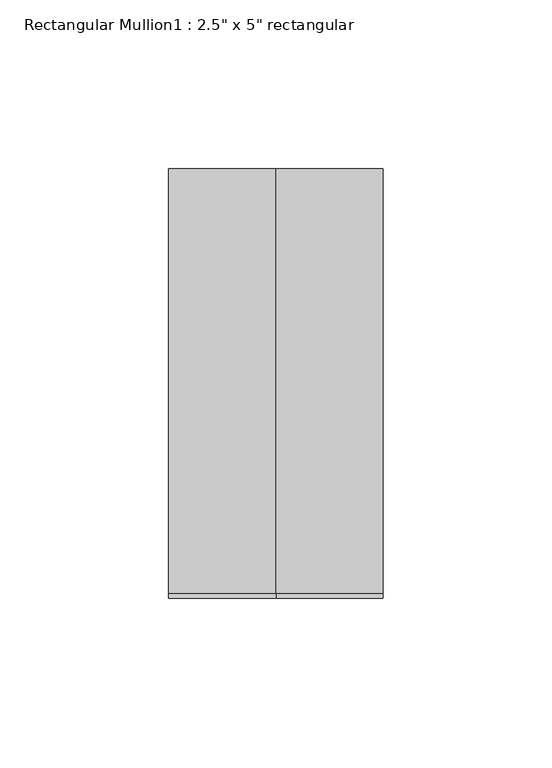
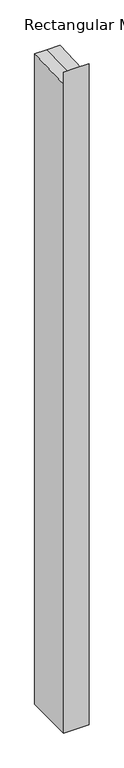
"""IFC4 building model written with IfcOpenShell, lengths in millimetres: member geometry."""

from ifc_helpers import new_model, si_unit, origin, place, context, project, spatial, faceted_brep, source, transform, mapped, element, save


def member_780b0c29(model_context):
    return source(origin(), model_context, "Body", "Brep", [
        faceted_brep([(31.75, 63.5, -1733.5500228), (31.75, -63.5, -1733.5500228), (-31.75, -63.5, -1733.5500228), (-31.75, 63.5, -1733.5500228), (-31.75, 63.5, 2.5257955), (0.0, 63.5, 2.5257955), (31.75, 63.5, 2.5257955), (-31.75, -63.5, 30.4748075), (-31.75, -62.1741259, -2.5237591), (31.75, -63.5, 30.4748075), (0.0, -63.5, 30.4748075), (31.75, -62.1741259, -2.5237591), (0.0, -62.1741259, -2.5237591)], [[[0, 1, 2, 3]], [[4, 5, 6, 0, 3]], [[7, 8, 4, 3, 2]], [[9, 10, 7, 2, 1]], [[6, 11, 9, 1, 0]], [[6, 5, 12, 11]], [[5, 4, 8, 12]], [[8, 7, 10, 12]], [[10, 9, 11, 12]]]),
    ])


if __name__ == "__main__":
    model = new_model("IFC4")
    model_context = context("Model", 3, world=origin())
    ifc_project = project(units=[si_unit("LENGTHUNIT", "METRE", prefix="MILLI")], contexts=[model_context])
    site = spatial("IfcSite", under=ifc_project)
    building = spatial("IfcBuilding", under=site)
    placement = place(None, origin())
    member_shape = member_780b0c29(model_context)
    element("IfcMember", 1, ObjectType="Rectangular Mullion1 : 2.5\" x 5\" rectangular", at=placement, inside=building, context=model_context, shape_type="MappedRepresentation", body=[
        mapped(member_shape, transform((0.0, 0.0, 0.0), x_axis=(1.0, 0.0, 0.0), y_axis=(0.0, 1.0, 0.0), z_axis=(0.0, 0.0, 1.0))),
    ])
    save(model, "model.ifc")

# Revit data of these elements
# Type "Rectangular Mullion1 : 2.5\" x 5\" rectangular"
#   built-in parameter 1007304 = 0.416667 (stored number, unit not read)
#   built-in parameter 1007301 = 0.104167 (stored number, unit not read)
#   built-in parameter 1007300 = 0.104167 (stored number, unit not read)
# Element 1 (IfcMember, "Rectangular Mullion1 : 2.5\" x 5\" rectangular")
#   Materials on its faces: "support-frame"
# Materials
#   "support-frame": class "Unassigned", colour RGB 233 233 233, transparency 0, Cost = 0
